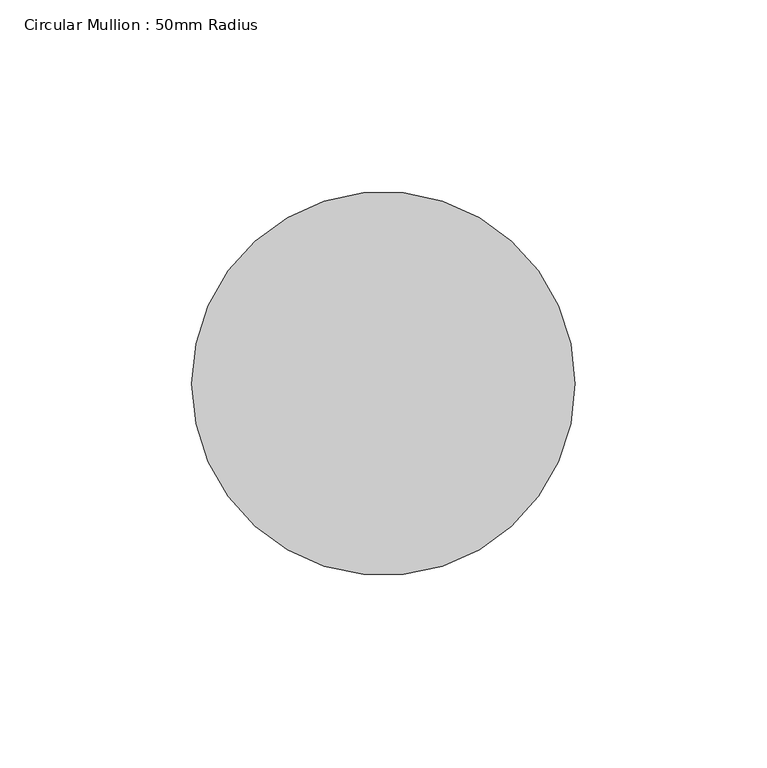
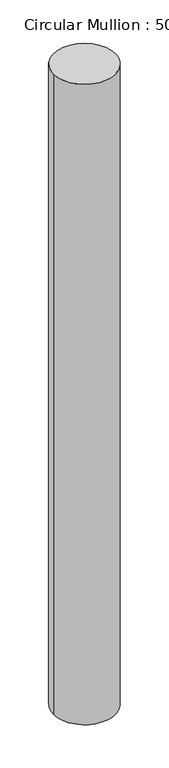
"""IFC4 building model written with IfcOpenShell, lengths in millimetres: member geometry, Circular Mullion : 50mm Radius."""

import ifcopenshell
import ifcopenshell.guid

model = None  # the IFC model being written
_history = None  # IfcOwnerHistory: only IFC2X3 demands one
_inside = {}  # id of a spatial element -> (the spatial element, [elements in it])
_under = {}  # id of a project, library or spatial element -> (it, [spatial elements below it])
_declared = {}  # id of a project -> (the project, [libraries it declares])
_typed = {}  # id of a type object -> (the type object, [elements of that type])
_made_of = {}  # id of a material, layer set ... -> (it, [elements and type objects made of it])


def new_model(schema):
    """Start an empty IFC model of exactly this schema.

    Asked for "IFC4X3", IfcOpenShell would pick the latest addendum, in which some entities
    have other attributes; the version numbers below select the first issue.
    IFC2X3 requires an IfcOwnerHistory on every rooted entity: one is made here for all.
    """
    global model, _history
    if schema == "IFC4X3":
        model = ifcopenshell.file(schema_version=(4, 3, 0, 0))
    else:
        model = ifcopenshell.file(schema=schema)
    _inside.clear()
    _under.clear()
    _declared.clear()
    _typed.clear()
    _made_of.clear()
    _history = None
    if model.schema == "IFC2X3":
        org = make("IfcOrganization", Name="unknown")
        user = make(
            "IfcPersonAndOrganization",
            ThePerson=make("IfcPerson", FamilyName="unknown"),
            TheOrganization=org,
        )
        app = make(
            "IfcApplication",
            ApplicationDeveloper=org,
            Version="unknown",
            ApplicationFullName="unknown",
            ApplicationIdentifier="unknown",
        )
        _history = make(
            "IfcOwnerHistory",
            OwningUser=user,
            OwningApplication=app,
            ChangeAction="ADDED",
            CreationDate=0,
        )
    return model


def make(cls, **values):
    """One entity of the class cls with the attributes given. An attribute that is None is left unset."""
    return model.create_entity(
        cls, **{name: value for name, value in values.items() if value is not None}
    )


def rooted(cls, **values):
    """An entity with a GlobalId (a new one), such as an element, a storey or a relation."""
    return make(cls, GlobalId=ifcopenshell.guid.new(), OwnerHistory=_history, **values)


def si_unit(unit_type, name, prefix=None):
    """IfcSIUnit, for example si_unit("LENGTHUNIT", "METRE", prefix="MILLI")."""
    return make("IfcSIUnit", UnitType=unit_type, Prefix=prefix, Name=name)


def assignment(units):
    """IfcUnitAssignment: the units of a project."""
    return None if units is None else make("IfcUnitAssignment", Units=units)


def point(xyz):
    """IfcCartesianPoint."""
    return None if xyz is None else make("IfcCartesianPoint", Coordinates=xyz)


def direction(xyz):
    """IfcDirection."""
    return None if xyz is None else make("IfcDirection", DirectionRatios=xyz)


def frame(location, z_axis=None, x_axis=None):
    """IfcAxis2Placement3D, a coordinate frame: its origin and axes. An axis left out is left unset."""
    return make(
        "IfcAxis2Placement3D",
        Location=point(location),
        Axis=direction(z_axis),
        RefDirection=direction(x_axis),
    )


def frame_2d(location, x_axis=None):
    """IfcAxis2Placement2D, a coordinate frame in the plane: its origin and x axis."""
    return make(
        "IfcAxis2Placement2D", Location=point(location), RefDirection=direction(x_axis)
    )


def origin():
    """The frame at (0, 0, 0) with its axes left unset."""
    return frame((0.0, 0.0, 0.0))


def origin_2d():
    """The frame at (0, 0) in the plane with its x axis left unset."""
    return frame_2d((0.0, 0.0))


def place(relative_to, where):
    """IfcLocalPlacement: puts the frame where relative to a parent placement (None: the world)."""
    return make(
        "IfcLocalPlacement", PlacementRelTo=relative_to, RelativePlacement=where
    )


def context(
    kind, dimensions, precision=None, world=None, true_north=None, identifier=None
):
    """IfcGeometricRepresentationContext, for example the 3D "Model" context."""
    return make(
        "IfcGeometricRepresentationContext",
        ContextIdentifier=identifier,
        ContextType=kind,
        CoordinateSpaceDimension=dimensions,
        Precision=precision,
        WorldCoordinateSystem=world,
        TrueNorth=true_north,
    )


def project(units=None, contexts=None):
    """IfcProject with its units and contexts."""
    return rooted(
        "IfcProject",
        Name="project",
        RepresentationContexts=contexts,
        UnitsInContext=assignment(units),
    )


def spatial(cls, under=None, at=None, **own):
    """A site, building, storey or space (cls), placed at a placement, below another one or the project."""
    s = rooted(cls, ObjectPlacement=at, **own)
    if under is not None:
        _under.setdefault(under.id(), (under, []))[1].append(s)
    return s


def circle_curve(where, radius):
    """IfcCircle in the frame where."""
    return make("IfcCircle", Position=where, Radius=radius)


def trimmed(basis, trim1, trim2, sense, master):
    """IfcTrimmedCurve: the piece of a basis curve between two trims."""
    return make(
        "IfcTrimmedCurve",
        BasisCurve=basis,
        Trim1=trim1,
        Trim2=trim2,
        SenseAgreement=sense,
        MasterRepresentation=master,
    )


def segment(curve, same_sense, transition):
    """IfcCompositeCurveSegment."""
    return make(
        "IfcCompositeCurveSegment",
        Transition=transition,
        SameSense=same_sense,
        ParentCurve=curve,
    )


def composite_curve(segments, self_intersect=None):
    """IfcCompositeCurve: segments joined end to end."""
    return make("IfcCompositeCurve", Segments=segments, SelfIntersect=self_intersect)


def outline(outer, holes=None, kind="AREA"):
    """IfcArbitraryClosedProfileDef: a profile drawn as a closed curve; with holes, ...WithVoids."""
    if holes is None:
        return make("IfcArbitraryClosedProfileDef", ProfileType=kind, OuterCurve=outer)
    return make(
        "IfcArbitraryProfileDefWithVoids",
        ProfileType=kind,
        OuterCurve=outer,
        InnerCurves=holes,
    )


def extrude(swept, where, along, depth):
    """IfcExtrudedAreaSolid: the profile swept, set in the frame where, extruded along a direction by depth."""
    return make(
        "IfcExtrudedAreaSolid",
        SweptArea=swept,
        Position=where,
        ExtrudedDirection=direction(along),
        Depth=depth,
    )


def shape(context_of_items, identifier, shape_type, items):
    """IfcShapeRepresentation: the items that make up one representation, for example the "Body"."""
    return make(
        "IfcShapeRepresentation",
        ContextOfItems=context_of_items,
        RepresentationIdentifier=identifier,
        RepresentationType=shape_type,
        Items=items,
    )


def source(mapping_origin, context_of_items, identifier, shape_type, items):
    """IfcRepresentationMap: a shape defined once, which mapped items show again and again."""
    return make(
        "IfcRepresentationMap",
        MappingOrigin=mapping_origin,
        MappedRepresentation=shape(context_of_items, identifier, shape_type, items),
    )


def transform(
    local_origin,
    x_axis=None,
    y_axis=None,
    z_axis=None,
    scale=None,
    scale2=None,
    scale3=None,
    uniform=True,
):
    """IfcCartesianTransformationOperator3D, or its non-uniform kind. x_axis, y_axis, z_axis: its Axis1, 2, 3."""
    if uniform:
        return make(
            "IfcCartesianTransformationOperator3D",
            Axis1=direction(x_axis),
            Axis2=direction(y_axis),
            LocalOrigin=point(local_origin),
            Scale=scale,
            Axis3=direction(z_axis),
        )
    return make(
        "IfcCartesianTransformationOperator3DnonUniform",
        Axis1=direction(x_axis),
        Axis2=direction(y_axis),
        LocalOrigin=point(local_origin),
        Scale=scale,
        Axis3=direction(z_axis),
        Scale2=scale2,
        Scale3=scale3,
    )


def mapped(mapping_source, mapping_target):
    """IfcMappedItem: shows the shape of a source again, moved by a transform."""
    return make(
        "IfcMappedItem", MappingSource=mapping_source, MappingTarget=mapping_target
    )


def made_of(thing, what):
    """Note that an element or type object is made of a material, layer set ...; save() writes the relation."""
    if what is not None:
        _made_of.setdefault(what.id(), (what, []))[1].append(thing)
    return thing


def element(
    cls,
    number,
    at=None,
    inside=None,
    cuts=None,
    type_object=None,
    material=None,
    context=None,
    identifier="Body",
    shape_type=None,
    held_by="IfcProductDefinitionShape",
    body=None,
    shapes=None,
    **own,
):
    """One element of the class cls, such as IfcWall. Its Tag is "e" and its number.

    at: its placement. inside: the storey or other place that contains it. cuts: it is an
    opening in that element (IfcRelVoidsElement). A single representation is given by context,
    identifier, shape_type and body (its items); several are given by shapes. held_by: the class
    of the entity that holds the representations. save() writes the other relations.
    """
    e = rooted(cls, Tag="e%d" % number, ObjectPlacement=at, **own)
    if body is not None:
        shapes = [shape(context, identifier, shape_type, body)]
    if shapes is not None:
        e.Representation = make(held_by, Representations=shapes)
    if inside is not None:
        _inside.setdefault(inside.id(), (inside, []))[1].append(e)
    if cuts is not None:
        rooted(
            "IfcRelVoidsElement", RelatingBuildingElement=cuts, RelatedOpeningElement=e
        )
    if type_object is not None:
        _typed.setdefault(type_object.id(), (type_object, []))[1].append(e)
    return made_of(e, material)


def aggregate(whole, parts):
    """IfcRelAggregates: a whole, such as a stair, and the parts it consists of."""
    return rooted("IfcRelAggregates", RelatingObject=whole, RelatedObjects=parts)


def save(model, path):
    """Write the relations noted so far, then the file.

    IfcRelAggregates (storeys below a building ...), IfcRelContainedInSpatialStructure (elements
    in a storey), IfcRelDefinesByType, IfcRelAssociatesMaterial and IfcRelDeclares: one each for
    every whole, place, type object, material and project.
    """
    for whole, parts in _under.values():
        aggregate(whole, parts)
    for where, things in _inside.values():
        rooted(
            "IfcRelContainedInSpatialStructure",
            RelatedElements=things,
            RelatingStructure=where,
        )
    for kind, things in _typed.values():
        rooted("IfcRelDefinesByType", RelatedObjects=things, RelatingType=kind)
    for what, things in _made_of.values():
        rooted("IfcRelAssociatesMaterial", RelatedObjects=things, RelatingMaterial=what)
    for by, libraries in _declared.values():
        rooted("IfcRelDeclares", RelatingContext=by, RelatedDefinitions=libraries)
    model.write(path)


def circular_mullion_50mm_radius_e59af530(model_context):
    return source(origin(), model_context, "Body", "SweptSolid", [
        extrude(outline(composite_curve([segment(trimmed(circle_curve(origin_2d(), 50.0), [point((50.0, 0.0))], [point((-50.0, 0.0))], False, "CARTESIAN"), True, "CONTINUOUS"), segment(trimmed(circle_curve(origin_2d(), 50.0), [point((-50.0, 0.0))], [point((50.0, 0.0))], False, "CARTESIAN"), True, "CONTINUOUS")], self_intersect=False)), frame((0.0, 0.0, -1092.0832038), z_axis=(0.0, 0.0, 1.0), x_axis=(1.0, 0.0, 0.0)), (0.0, 0.0, 1.0), 1092.0832038),
    ])


if __name__ == "__main__":
    model = new_model("IFC4")
    model_context = context("Model", 3, world=origin())
    ifc_project = project(units=[si_unit("LENGTHUNIT", "METRE", prefix="MILLI")], contexts=[model_context])
    site = spatial("IfcSite", under=ifc_project)
    building = spatial("IfcBuilding", under=site)
    placement = place(None, origin())
    circular_mullion_50mm_radius_shape = circular_mullion_50mm_radius_e59af530(model_context)
    element("IfcMember", 1, ObjectType="Circular Mullion : 50mm Radius", at=placement, inside=building, context=model_context, shape_type="MappedRepresentation", body=[
        mapped(circular_mullion_50mm_radius_shape, transform((0.0, 0.0, 0.0), x_axis=(1.0, 0.0, 0.0), y_axis=(0.0, 1.0, 0.0), z_axis=(0.0, 0.0, 1.0))),
    ])
    save(model, "model.ifc")

# Revit data of these elements
# Type "Circular Mullion : 50mm Radius"
#   built-in parameter 1007350 = 0.164042 (stored number, unit not read)
# Element 1 (IfcMember, "Circular Mullion : 50mm Radius")
#   Materials on its faces: "Aluminium"
# Materials
#   "Aluminium": class "Metal", colour RGB 247 247 247, transparency 0, Description = "Aluminium 6061", Cost = 0
